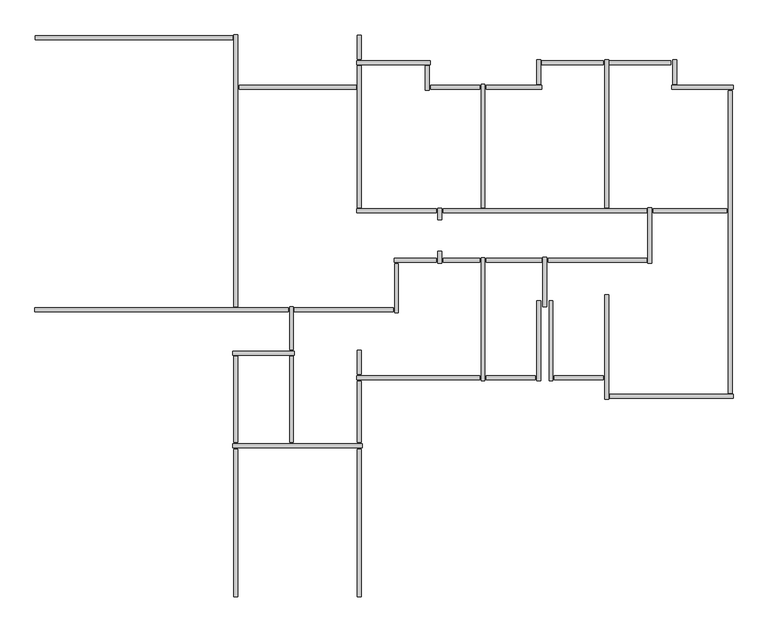
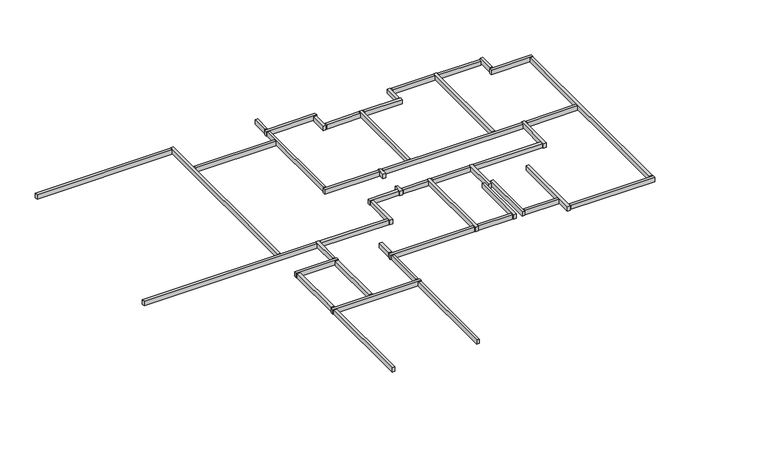
"""IFC4 building model written with IfcOpenShell, lengths in millimetres: beam geometry, Graute viga de respaldo9 : Graute viga de respaldo."""

from ifc_helpers import new_model, si_unit, frame, origin, place, context, project, spatial, polyline, outline, extrude, source, transform, mapped, element, save


def beam_2cfba711(model_context):
    return source(origin(), model_context, "Body", "SweptSolid", [
        extrude(outline(polyline([(-62804.9587292, 72814.9577736), (-62804.9587292, 72720.9577736), (-67594.9587292, 72720.9577736), (-67594.9587292, 72814.9577736), (-62804.9587292, 72814.9577736)])), frame((0.0, 0.0, 8632.9999999), z_axis=(0.0, 0.0, 1.0), x_axis=(1.0, 0.0, 0.0)), (0.0, 0.0, 1.0), 167.0),
        extrude(outline(polyline([(-59771.9587292, 62785.4278788), (-59677.9587292, 62785.4278788), (-59677.9587292, 59195.4278788), (-59771.9587292, 59195.4278788), (-59771.9587292, 62785.4278788)])), frame((0.0, 0.0, 8632.9999999), z_axis=(0.0, 0.0, 1.0), x_axis=(1.0, 0.0, 0.0)), (0.0, 0.0, 1.0), 167.0),
        extrude(outline(polyline([(-62771.9587292, 62785.4278788), (-62677.9587292, 62785.4278788), (-62677.9587292, 59195.4278788), (-62771.9587292, 59195.4278788), (-62771.9587292, 62785.4278788)])), frame((0.0, 0.0, 8632.9999999), z_axis=(0.0, 0.0, 1.0), x_axis=(1.0, 0.0, 0.0)), (0.0, 0.0, 1.0), 167.0),
        extrude(outline(polyline([(-54994.9587292, 64468.4278788), (-54994.9587292, 64562.4278788), (-53804.9587292, 64562.4278788), (-53804.9587292, 64468.4278788), (-54994.9587292, 64468.4278788)])), frame((0.0, 0.0, 8632.9999999), z_axis=(0.0, 0.0, 1.0), x_axis=(1.0, 0.0, 0.0)), (0.0, 0.0, 1.0), 167.0),
        extrude(outline(polyline([(-56644.9587292, 64468.4278788), (-56644.9587292, 64562.4278788), (-55454.9587292, 64562.4278788), (-55454.9587292, 64468.4278788), (-56644.9587292, 64468.4278788)])), frame((0.0, 0.0, 8632.9999999), z_axis=(0.0, 0.0, 1.0), x_axis=(1.0, 0.0, 0.0)), (0.0, 0.0, 1.0), 167.0),
        extrude(outline(polyline([(-52594.9587292, 68518.4278788), (-52594.9587292, 68612.4278788), (-50804.9587292, 68612.4278788), (-50804.9587292, 68518.4278788), (-52594.9587292, 68518.4278788)])), frame((0.0, 0.0, 8632.9999999), z_axis=(0.0, 0.0, 1.0), x_axis=(1.0, 0.0, 0.0)), (0.0, 0.0, 1.0), 167.0),
        extrude(outline(polyline([(-57994.9587292, 71518.4278788), (-57994.9587292, 71612.4278788), (-56804.9587292, 71612.4278788), (-56804.9587292, 71518.4278788), (-57994.9587292, 71518.4278788)])), frame((0.0, 0.0, 8632.9999999), z_axis=(0.0, 0.0, 1.0), x_axis=(1.0, 0.0, 0.0)), (0.0, 0.0, 1.0), 167.0),
        extrude(outline(polyline([(-58027.9587292, 71495.4278788), (-58121.9587292, 71495.4278788), (-58121.9587292, 72085.4278788), (-58027.9587292, 72085.4278788), (-58027.9587292, 71495.4278788)])), frame((0.0, 0.0, 8632.9999999), z_axis=(0.0, 0.0, 1.0), x_axis=(1.0, 0.0, 0.0)), (0.0, 0.0, 1.0), 167.0),
        extrude(outline(polyline([(-59794.9587292, 72118.4278788), (-59794.9587292, 72212.4278788), (-58004.9587292, 72212.4278788), (-58004.9587292, 72118.4278788), (-59794.9587292, 72118.4278788)])), frame((0.0, 0.0, 8632.9999999), z_axis=(0.0, 0.0, 1.0), x_axis=(1.0, 0.0, 0.0)), (0.0, 0.0, 1.0), 167.0),
        extrude(outline(polyline([(-57821.9587292, 68635.4278788), (-57727.9587292, 68635.4278788), (-57727.9587292, 68345.4278788), (-57821.9587292, 68345.4278788), (-57821.9587292, 68635.4278788)])), frame((0.0, 0.0, 8632.9999999), z_axis=(0.0, 0.0, 1.0), x_axis=(1.0, 0.0, 0.0)), (0.0, 0.0, 1.0), 167.0),
        extrude(outline(polyline([(-55144.9587292, 67318.4278788), (-55144.9587292, 67412.4278788), (-52754.9587292, 67412.4278788), (-52754.9587292, 67318.4278788), (-55144.9587292, 67318.4278788)])), frame((0.0, 0.0, 8632.9999999), z_axis=(0.0, 0.0, 1.0), x_axis=(1.0, 0.0, 0.0)), (0.0, 0.0, 1.0), 167.0),
        extrude(outline(polyline([(-56644.9587292, 67318.4278788), (-56644.9587292, 67412.4278788), (-55304.9587292, 67412.4278788), (-55304.9587292, 67318.4278788), (-56644.9587292, 67318.4278788)])), frame((0.0, 0.0, 8632.9999999), z_axis=(0.0, 0.0, 1.0), x_axis=(1.0, 0.0, 0.0)), (0.0, 0.0, 1.0), 167.0),
        extrude(outline(polyline([(-57694.9587292, 67318.4278788), (-57694.9587292, 67412.4278788), (-56804.9587292, 67412.4278788), (-56804.9587292, 67318.4278788), (-57694.9587292, 67318.4278788)])), frame((0.0, 0.0, 8632.9999999), z_axis=(0.0, 0.0, 1.0), x_axis=(1.0, 0.0, 0.0)), (0.0, 0.0, 1.0), 167.0),
        extrude(outline(polyline([(-57821.9587292, 67585.4278788), (-57727.9587292, 67585.4278788), (-57727.9587292, 67295.4278788), (-57821.9587292, 67295.4278788), (-57821.9587292, 67585.4278788)])), frame((0.0, 0.0, 8632.9999999), z_axis=(0.0, 0.0, 1.0), x_axis=(1.0, 0.0, 0.0)), (0.0, 0.0, 1.0), 167.0),
        extrude(outline(polyline([(-58884.9587292, 67318.4278788), (-58884.9587292, 67412.4278788), (-57854.9587292, 67412.4278788), (-57854.9587292, 67318.4278788), (-58884.9587292, 67318.4278788)])), frame((0.0, 0.0, 8632.9999999), z_axis=(0.0, 0.0, 1.0), x_axis=(1.0, 0.0, 0.0)), (0.0, 0.0, 1.0), 167.0),
        extrude(outline(polyline([(-58777.9587292, 66095.4278788), (-58871.9587292, 66095.4278788), (-58871.9587292, 67285.4278788), (-58777.9587292, 67285.4278788), (-58777.9587292, 66095.4278788)])), frame((0.0, 0.0, 8632.9999999), z_axis=(0.0, 0.0, 1.0), x_axis=(1.0, 0.0, 0.0)), (0.0, 0.0, 1.0), 167.0),
        extrude(outline(polyline([(-61304.9587292, 66118.4278788), (-61304.9587292, 66212.4278788), (-58904.9587292, 66212.4278788), (-58904.9587292, 66118.4278788), (-61304.9587292, 66118.4278788)])), frame((0.0, 0.0, 8632.9999999), z_axis=(0.0, 0.0, 1.0), x_axis=(1.0, 0.0, 0.0)), (0.0, 0.0, 1.0), 167.0),
        extrude(outline(polyline([(-56771.9587292, 67430.4278788), (-56677.9587292, 67430.4278788), (-56677.9587292, 64445.4278788), (-56771.9587292, 64445.4278788), (-56771.9587292, 67430.4278788)])), frame((0.0, 0.0, 8632.9999999), z_axis=(0.0, 0.0, 1.0), x_axis=(1.0, 0.0, 0.0)), (0.0, 0.0, 1.0), 167.0),
        extrude(outline(polyline([(-59794.9587292, 64468.4278788), (-59794.9587292, 64562.4278788), (-56804.9587292, 64562.4278788), (-56804.9587292, 64468.4278788), (-59794.9587292, 64468.4278788)])), frame((0.0, 0.0, 8632.9999999), z_axis=(0.0, 0.0, 1.0), x_axis=(1.0, 0.0, 0.0)), (0.0, 0.0, 1.0), 167.0),
        extrude(outline(polyline([(-59771.9587292, 65185.4278788), (-59677.9587292, 65185.4278788), (-59677.9587292, 64595.4278788), (-59771.9587292, 64595.4278788), (-59771.9587292, 65185.4278788)])), frame((0.0, 0.0, 8632.9999999), z_axis=(0.0, 0.0, 1.0), x_axis=(1.0, 0.0, 0.0)), (0.0, 0.0, 1.0), 167.0),
        extrude(outline(polyline([(-59677.9587292, 62945.4278788), (-59771.9587292, 62945.4278788), (-59771.9587292, 64435.4278788), (-59677.9587292, 64435.4278788), (-59677.9587292, 62945.4278788)])), frame((0.0, 0.0, 8632.9999999), z_axis=(0.0, 0.0, 1.0), x_axis=(1.0, 0.0, 0.0)), (0.0, 0.0, 1.0), 167.0),
        extrude(outline(polyline([(-62677.9587292, 62945.4278788), (-62771.9587292, 62945.4278788), (-62771.9587292, 65035.4278788), (-62677.9587292, 65035.4278788), (-62677.9587292, 62945.4278788)])), frame((0.0, 0.0, 8632.9999999), z_axis=(0.0, 0.0, 1.0), x_axis=(1.0, 0.0, 0.0)), (0.0, 0.0, 1.0), 167.0),
        extrude(outline(polyline([(-61327.9587292, 62945.4278788), (-61421.9587292, 62945.4278788), (-61421.9587292, 65035.4278788), (-61327.9587292, 65035.4278788), (-61327.9587292, 62945.4278788)])), frame((0.0, 0.0, 8632.9999999), z_axis=(0.0, 0.0, 1.0), x_axis=(1.0, 0.0, 0.0)), (0.0, 0.0, 1.0), 167.0),
        extrude(outline(polyline([(-61421.9587292, 66235.4278788), (-61327.9587292, 66235.4278788), (-61327.9587292, 65195.4278788), (-61421.9587292, 65195.4278788), (-61421.9587292, 66235.4278788)])), frame((0.0, 0.0, 8632.9999999), z_axis=(0.0, 0.0, 1.0), x_axis=(1.0, 0.0, 0.0)), (0.0, 0.0, 1.0), 167.0),
        extrude(outline(polyline([(-62644.9587292, 71518.4278788), (-62644.9587292, 71612.4278788), (-59804.9587292, 71612.4278788), (-59804.9587292, 71518.4278788), (-62644.9587292, 71518.4278788)])), frame((0.0, 0.0, 8632.9999999), z_axis=(0.0, 0.0, 1.0), x_axis=(1.0, 0.0, 0.0)), (0.0, 0.0, 1.0), 167.0),
        extrude(outline(polyline([(-59677.9587292, 68645.4278788), (-59771.9587292, 68645.4278788), (-59771.9587292, 72085.4278788), (-59677.9587292, 72085.4278788), (-59677.9587292, 68645.4278788)])), frame((0.0, 0.0, 8632.9999999), z_axis=(0.0, 0.0, 1.0), x_axis=(1.0, 0.0, 0.0)), (0.0, 0.0, 1.0), 167.0),
        extrude(outline(polyline([(-59794.9587292, 68518.4278788), (-59794.9587292, 68612.4278788), (-57854.9587292, 68612.4278788), (-57854.9587292, 68518.4278788), (-59794.9587292, 68518.4278788)])), frame((0.0, 0.0, 8632.9999999), z_axis=(0.0, 0.0, 1.0), x_axis=(1.0, 0.0, 0.0)), (0.0, 0.0, 1.0), 167.0),
        extrude(outline(polyline([(-57694.9587292, 68518.4278788), (-57694.9587292, 68612.4278788), (-52754.9587292, 68612.4278788), (-52754.9587292, 68518.4278788), (-57694.9587292, 68518.4278788)])), frame((0.0, 0.0, 8632.9999999), z_axis=(0.0, 0.0, 1.0), x_axis=(1.0, 0.0, 0.0)), (0.0, 0.0, 1.0), 167.0),
        extrude(outline(polyline([(-56771.9587292, 71635.4278788), (-56677.9587292, 71635.4278788), (-56677.9587292, 68645.4278788), (-56771.9587292, 68645.4278788), (-56771.9587292, 71635.4278788)])), frame((0.0, 0.0, 8632.9999999), z_axis=(0.0, 0.0, 1.0), x_axis=(1.0, 0.0, 0.0)), (0.0, 0.0, 1.0), 167.0),
        extrude(outline(polyline([(-55304.9587292, 71612.4278788), (-55304.9587292, 71518.4278788), (-56644.9587292, 71518.4278788), (-56644.9587292, 71612.4278788), (-55304.9587292, 71612.4278788)])), frame((0.0, 0.0, 8632.9999999), z_axis=(0.0, 0.0, 1.0), x_axis=(1.0, 0.0, 0.0)), (0.0, 0.0, 1.0), 167.0),
        extrude(outline(polyline([(-55421.9587292, 72235.4278788), (-55327.9587292, 72235.4278788), (-55327.9587292, 71645.4278788), (-55421.9587292, 71645.4278788), (-55421.9587292, 72235.4278788)])), frame((0.0, 0.0, 8632.9999999), z_axis=(0.0, 0.0, 1.0), x_axis=(1.0, 0.0, 0.0)), (0.0, 0.0, 1.0), 167.0),
        extrude(outline(polyline([(-55294.9587292, 72118.4278788), (-55294.9587292, 72212.4278788), (-53804.9587292, 72212.4278788), (-53804.9587292, 72118.4278788), (-55294.9587292, 72118.4278788)])), frame((0.0, 0.0, 8632.9999999), z_axis=(0.0, 0.0, 1.0), x_axis=(1.0, 0.0, 0.0)), (0.0, 0.0, 1.0), 167.0),
        extrude(outline(polyline([(-52165.9809043, 72212.4278788), (-52165.9809043, 72117.4278788), (-53654.9587292, 72117.4278788), (-53654.9587292, 72212.4278788), (-52165.9809043, 72212.4278788)])), frame((0.0, 0.0, 8617.1856208), z_axis=(0.0, 0.0, 1.0), x_axis=(1.0, 0.0, 0.0)), (0.0, 0.0, 1.0), 165.0),
        extrude(outline(polyline([(-50677.9587292, 64145.4278788), (-50771.9587292, 64145.4278788), (-50771.9587292, 71485.4278788), (-50677.9587292, 71485.4278788), (-50677.9587292, 64145.4278788)])), frame((0.0, 0.0, 8632.9999999), z_axis=(0.0, 0.0, 1.0), x_axis=(1.0, 0.0, 0.0)), (0.0, 0.0, 1.0), 167.0),
        extrude(outline(polyline([(-52627.9587292, 67295.4278788), (-52721.9587292, 67295.4278788), (-52721.9587292, 68640.7810915), (-52627.9587292, 68640.7810915), (-52627.9587292, 67295.4278788)])), frame((0.0, 0.0, 8632.9999999), z_axis=(0.0, 0.0, 1.0), x_axis=(1.0, 0.0, 0.0)), (0.0, 0.0, 1.0), 167.0),
        extrude(outline(polyline([(-55177.9587292, 66245.4278788), (-55271.9587292, 66245.4278788), (-55271.9587292, 67435.4278788), (-55177.9587292, 67435.4278788), (-55177.9587292, 66245.4278788)])), frame((0.0, 0.0, 8632.9999999), z_axis=(0.0, 0.0, 1.0), x_axis=(1.0, 0.0, 0.0)), (0.0, 0.0, 1.0), 167.0),
        extrude(outline(polyline([(-55027.9587292, 64445.4278788), (-55121.9587292, 64445.4278788), (-55121.9587292, 66385.4278788), (-55027.9587292, 66385.4278788), (-55027.9587292, 64445.4278788)])), frame((0.0, 0.0, 8632.9999999), z_axis=(0.0, 0.0, 1.0), x_axis=(1.0, 0.0, 0.0)), (0.0, 0.0, 1.0), 167.0),
        extrude(outline(polyline([(-55327.9587292, 64445.4278788), (-55421.9587292, 64445.4278788), (-55421.9587292, 66385.4278788), (-55327.9587292, 66385.4278788), (-55327.9587292, 64445.4278788)])), frame((0.0, 0.0, 8632.9999999), z_axis=(0.0, 0.0, 1.0), x_axis=(1.0, 0.0, 0.0)), (0.0, 0.0, 1.0), 167.0),
        extrude(outline(polyline([(-53677.9587292, 63995.4278788), (-53771.9587292, 63995.4278788), (-53771.9587292, 66535.4278788), (-53677.9587292, 66535.4278788), (-53677.9587292, 63995.4278788)])), frame((0.0, 0.0, 8632.9999999), z_axis=(0.0, 0.0, 1.0), x_axis=(1.0, 0.0, 0.0)), (0.0, 0.0, 1.0), 167.0),
        extrude(outline(polyline([(-50654.9587292, 64112.4278788), (-50654.9587292, 64018.4278788), (-53644.9587292, 64018.4278788), (-53644.9587292, 64112.4278788), (-50654.9587292, 64112.4278788)])), frame((0.0, 0.0, 8632.9999999), z_axis=(0.0, 0.0, 1.0), x_axis=(1.0, 0.0, 0.0)), (0.0, 0.0, 1.0), 167.0),
        extrude(outline(polyline([(-52121.9587292, 72235.4278788), (-52027.9587292, 72235.4278788), (-52027.9587292, 71645.4278788), (-52121.9587292, 71645.4278788), (-52121.9587292, 72235.4278788)])), frame((0.0, 0.0, 8632.9999999), z_axis=(0.0, 0.0, 1.0), x_axis=(1.0, 0.0, 0.0)), (0.0, 0.0, 1.0), 167.0),
        extrude(outline(polyline([(-52144.9587292, 71518.4278788), (-52144.9587292, 71612.4278788), (-50654.9587292, 71612.4278788), (-50654.9587292, 71518.4278788), (-52144.9587292, 71518.4278788)])), frame((0.0, 0.0, 8632.9999999), z_axis=(0.0, 0.0, 1.0), x_axis=(1.0, 0.0, 0.0)), (0.0, 0.0, 1.0), 167.0),
        extrude(outline(polyline([(-53771.9587292, 72235.4278788), (-53677.9587292, 72235.4278788), (-53677.9587292, 68645.4278788), (-53771.9587292, 68645.4278788), (-53771.9587292, 72235.4278788)])), frame((0.0, 0.0, 8632.9999999), z_axis=(0.0, 0.0, 1.0), x_axis=(1.0, 0.0, 0.0)), (0.0, 0.0, 1.0), 167.0),
        extrude(outline(polyline([(-59771.9587292, 72835.4278788), (-59677.9587292, 72835.4278788), (-59677.9587292, 72245.4278788), (-59771.9587292, 72245.4278788), (-59771.9587292, 72835.4278788)])), frame((0.0, 0.0, 8632.9999999), z_axis=(0.0, 0.0, 1.0), x_axis=(1.0, 0.0, 0.0)), (0.0, 0.0, 1.0), 167.0),
        extrude(outline(polyline([(-62794.9587292, 65068.4278788), (-62794.9587292, 65162.4278788), (-61304.9587292, 65162.4278788), (-61304.9587292, 65068.4278788), (-62794.9587292, 65068.4278788)])), frame((0.0, 0.0, 8632.9999999), z_axis=(0.0, 0.0, 1.0), x_axis=(1.0, 0.0, 0.0)), (0.0, 0.0, 1.0), 167.0),
        extrude(outline(polyline([(-62794.9587292, 62818.4278788), (-62794.9587292, 62912.4278788), (-59654.9587292, 62912.4278788), (-59654.9587292, 62818.4278788), (-62794.9587292, 62818.4278788)])), frame((0.0, 0.0, 8632.9999999), z_axis=(0.0, 0.0, 1.0), x_axis=(1.0, 0.0, 0.0)), (0.0, 0.0, 1.0), 167.0),
        extrude(outline(polyline([(-67601.7587292, 66118.4278788), (-67601.7587292, 66212.4278788), (-61454.9587292, 66212.4278788), (-61454.9587292, 66118.4278788), (-67601.7587292, 66118.4278788)])), frame((0.0, 0.0, 8632.9999999), z_axis=(0.0, 0.0, 1.0), x_axis=(1.0, 0.0, 0.0)), (0.0, 0.0, 1.0), 167.0),
        extrude(outline(polyline([(-62771.9587292, 72837.9577736), (-62677.9587292, 72837.9577736), (-62677.9587292, 66245.4278788), (-62771.9587292, 66245.4278788), (-62771.9587292, 72837.9577736)])), frame((0.0, 0.0, 8632.9999999), z_axis=(0.0, 0.0, 1.0), x_axis=(1.0, 0.0, 0.0)), (0.0, 0.0, 1.0), 167.0),
    ])


if __name__ == "__main__":
    model = new_model("IFC4")
    model_context = context("Model", 3, world=origin())
    ifc_project = project(units=[si_unit("LENGTHUNIT", "METRE", prefix="MILLI")], contexts=[model_context])
    site = spatial("IfcSite", under=ifc_project)
    building = spatial("IfcBuilding", under=site)
    placement = place(None, origin())
    beam_shape = beam_2cfba711(model_context)
    element("IfcBeam", 1, ObjectType="Graute viga de respaldo9 : Graute viga de respaldo", at=placement, inside=building, context=model_context, shape_type="MappedRepresentation", body=[
        mapped(beam_shape, transform((0.0, 0.0, 0.0), x_axis=(1.0, 0.0, 0.0), y_axis=(0.0, 1.0, 0.0), z_axis=(0.0, 0.0, 1.0))),
    ])
    save(model, "model.ifc")

# Revit data of these elements
# Element 1 (IfcBeam, "Graute viga de respaldo9 : Graute viga de respaldo")
#   Materials on its faces: "Concreto, Faixa de areia/cimento"
# Materials
#   "Concreto, Faixa de areia/cimento": class "Concreto", colour RGB 127 127 127, transparency 0, Description = "Revestimento de laje de concreto", Cost = 0
